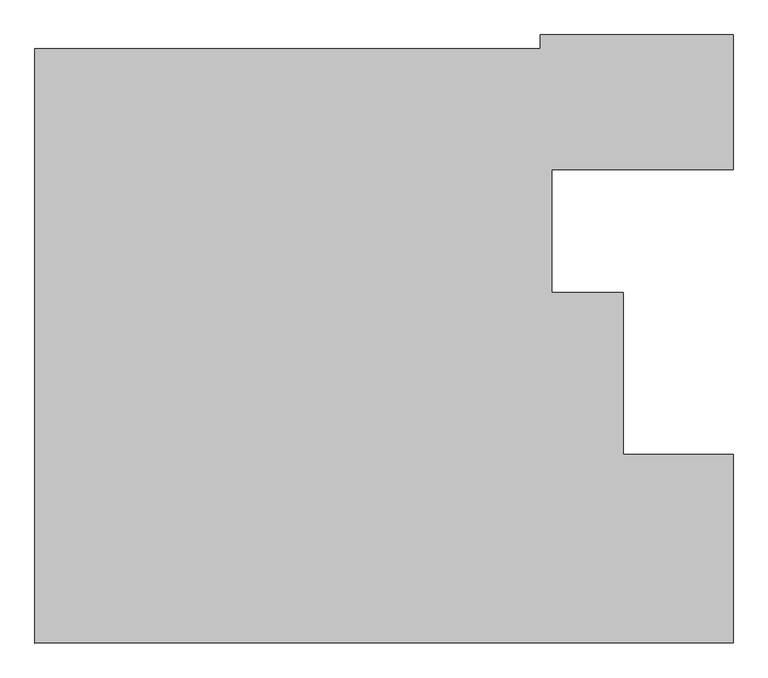
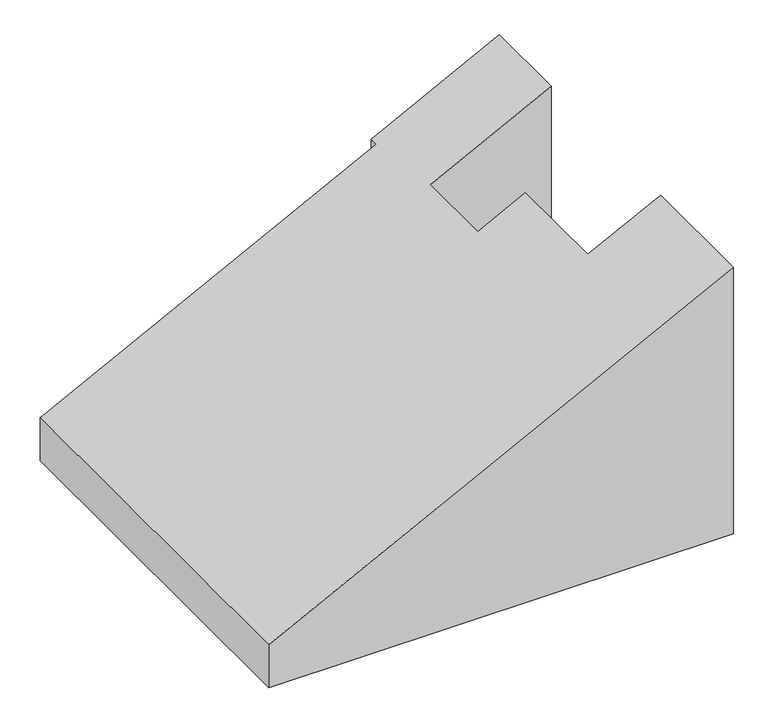
"""IFC4 building model written with IfcOpenShell, lengths in millimetres: proxy geometry, 0_3d."""

from ifc_helpers import new_model, si_unit, origin, place, context, project, spatial, faceted_brep, source, transform, mapped, element, save


def generic_models_67903bf8(model_context):
    return source(origin(), model_context, "Body", "Brep", [
        faceted_brep([(4720.0, 5552.8619019, 3043.5797924), (0.0, 5552.8619019, 638.6196708), (0.0, 0.0, 638.6196708), (6520.0, 0.0, 3960.7256015), (6520.0, 1763.2600653, 3960.7256015), (5495.0, 1763.2600653, 3438.4620158), (5495.0, 3272.8619019, 3438.4620158), (4825.0, 3272.8619019, 3097.0799646), (4825.0, 4422.8619019, 3097.0799646), (6520.0, 4422.8619019, 3960.7256015), (6520.0, 5682.8619019, 3960.7256015), (4720.0, 5682.8619019, 3043.5797924), (5495.0, 3272.8619019, 0.0), (4825.0, 3272.8619019, 0.0), (5495.0, 1763.2600653, 0.0), (6520.0, 1763.2600653, 0.0), (0.0, 0.0, 0.0), (6520.0, 0.0, 0.0), (0.0, 5552.8619019, 0.0), (4720.0, 5552.8619019, 0.0), (4720.0, 5682.8619019, 0.0), (6520.0, 5682.8619019, 0.0), (6520.0, 4422.8619019, 0.0), (4825.0, 4422.8619019, 0.0)], [[[0, 1, 2, 3, 4, 5, 6, 7, 8, 9, 10, 11]], [[7, 6, 12, 13]], [[6, 5, 14, 12]], [[5, 4, 15, 14]], [[3, 2, 16, 17]], [[2, 1, 18, 16]], [[1, 0, 19, 18]], [[0, 11, 20, 19]], [[11, 10, 21, 20]], [[22, 21, 10, 9]], [[9, 8, 23, 22]], [[8, 7, 13, 23]], [[17, 15, 4, 3]], [[16, 18, 19, 20, 21, 22, 23, 13, 12, 14, 15, 17]]]),
    ])


if __name__ == "__main__":
    model = new_model("IFC4")
    model_context = context("Model", 3, world=origin())
    ifc_project = project(units=[si_unit("LENGTHUNIT", "METRE", prefix="MILLI")], contexts=[model_context])
    site = spatial("IfcSite", under=ifc_project)
    building = spatial("IfcBuilding", under=site)
    placement = place(None, origin())
    generic_models_shape = generic_models_67903bf8(model_context)
    element("IfcBuildingElementProxy", 1, Name="0_3d", ObjectType="0_3d", at=placement, inside=building, context=model_context, shape_type="MappedRepresentation", body=[
        mapped(generic_models_shape, transform((0.0, 0.0, 0.0), x_axis=(1.0, 0.0, 0.0), y_axis=(0.0, 1.0, 0.0), z_axis=(0.0, 0.0, 1.0))),
    ])
    save(model, "model.ifc")

# Revit data of these elements
# Element 1 (IfcBuildingElementProxy, "0_3d")
#   Materials on its faces: "*1"
# Materials
#   "*1": class "Unassigned", colour RGB 175 175 175, transparency 0
